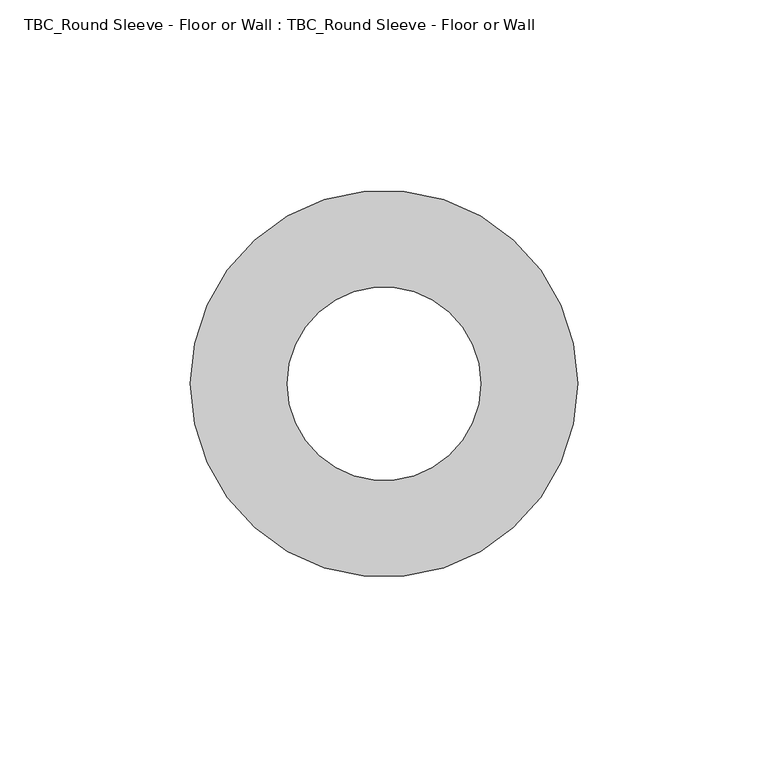
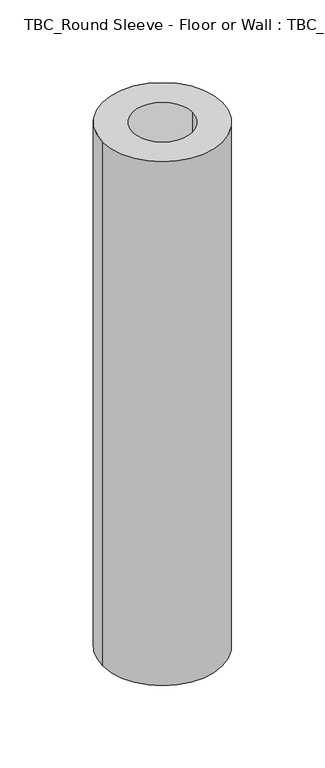
"""IFC4 building model written with IfcOpenShell, lengths in millimetres: proxy geometry, TBC_Round Sleeve - Floor or Wall : TBC_Round Sleeve - Floor or Wall."""

from ifc_helpers import new_model, si_unit, point, frame, origin, origin_2d, place, context, project, spatial, circle_curve, trimmed, segment, composite_curve, outline, extrude, source, transform, mapped, element, save


def tbc_round_sleeve_floor_or_wall_tbc_round_sleeve_floor_or_5e24f8f3(model_context):
    return source(origin(), model_context, "Body", "SweptSolid", [
        extrude(outline(composite_curve([segment(trimmed(circle_curve(origin_2d(), 50.8), [point((-50.8, 0.0))], [point((50.8, 0.0))], False, "CARTESIAN"), True, "CONTINUOUS"), segment(trimmed(circle_curve(origin_2d(), 50.8), [point((50.8, 0.0))], [point((-50.8, 0.0))], False, "CARTESIAN"), True, "CONTINUOUS")], self_intersect=False), holes=[composite_curve([segment(trimmed(circle_curve(origin_2d(), 25.4), [point((-25.4, 0.0))], [point((25.4, 0.0))], True, "CARTESIAN"), True, "CONTINUOUS"), segment(trimmed(circle_curve(origin_2d(), 25.4), [point((25.4, 0.0))], [point((-25.4, 0.0))], True, "CARTESIAN"), True, "CONTINUOUS")], self_intersect=False)]), frame((0.0, 0.0, -469.9), z_axis=(0.0, 0.0, 1.0), x_axis=(1.0, 0.0, 0.0)), (0.0, 0.0, 1.0), 469.9),
    ])


if __name__ == "__main__":
    model = new_model("IFC4")
    model_context = context("Model", 3, world=origin())
    ifc_project = project(units=[si_unit("LENGTHUNIT", "METRE", prefix="MILLI")], contexts=[model_context])
    site = spatial("IfcSite", under=ifc_project)
    building = spatial("IfcBuilding", under=site)
    placement = place(None, origin())
    tbc_round_sleeve_floor_or_wall_tbc_round_sleeve_floor_or_shape = tbc_round_sleeve_floor_or_wall_tbc_round_sleeve_floor_or_5e24f8f3(model_context)
    element("IfcBuildingElementProxy", 1, Name="TBC_Round Sleeve - Floor or Wall : TBC_Round Sleeve - Floor or Wall", ObjectType="TBC_Round Sleeve - Floor or Wall : TBC_Round Sleeve - Floor or Wall", at=placement, inside=building, context=model_context, shape_type="MappedRepresentation", body=[
        mapped(tbc_round_sleeve_floor_or_wall_tbc_round_sleeve_floor_or_shape, transform((0.0, 0.0, 0.0), x_axis=(1.0, 0.0, 0.0), y_axis=(0.0, 1.0, 0.0), z_axis=(0.0, 0.0, 1.0))),
    ])
    save(model, "model.ifc")

# Revit data of these elements
# Type "TBC_Round Sleeve - Floor or Wall : TBC_Round Sleeve - Floor or Wall"
#   Tag Dimension [instance default] = ""
#   MEP Type [instance default] = ""
#   MEP Element [instance default] = ""
#   MEP Category [instance default] = ""
#   Host Element Type [instance default] = ""
#   Host Element Id [instance default] = ""
#   Host Element Category [instance default] = ""
#   Control Line Y [instance default] = ""
#   Control Line X [instance default] = ""
#   Sleeve Radius [instance default] = 1' - 0"
#   Sleeve Edge [instance default] = 1' - 2"
#   Sleeve Depth [instance default] = 3' - 0"
#   Distance Y [instance default] = 0' - 0"
#   Distance X [instance default] = 0' - 0"
#   Default Elevation = 0
# Element 1 (IfcBuildingElementProxy, "TBC_Round Sleeve - Floor or Wall : TBC_Round Sleeve - Floor or Wall")
#   Tag Dimension = "2\"ø"
#   MEP Type = "PLG-G"
#   MEP Element = "898860"
#   MEP Category = "Pipe"
#   Host Element Type = "Roof Plank-Sleeves"
#   Host Element Id = "1525183"
#   Host Element Category = "Floors"
#   Sleeve Radius = 0' - 2"
#   Sleeve Edge = 0' - 4"
#   Sleeve Depth = 1' - 6 1/2"
